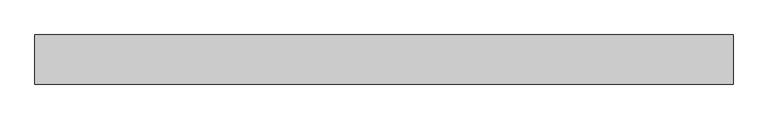
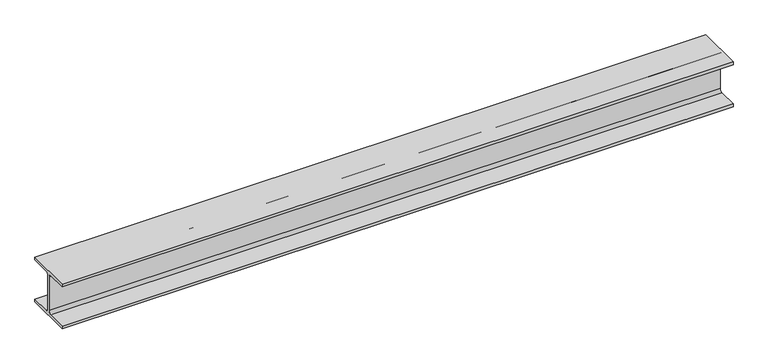
"""IFC4 building model written with IfcOpenShell, lengths in millimetres: beam geometry, 0912_Steel Framing_H-KSD3502 : H_SB_ASB_H-200x200x8x12."""

from ifc_helpers import new_model, si_unit, point, frame, frame_2d, origin, place, context, project, spatial, polyline, circle_curve, trimmed, segment, composite_curve, outline, extrude, source, transform, mapped, element, save


def beam_16896ac0(model_context):
    return source(origin(), model_context, "Body", "SweptSolid", [
        extrude(outline(composite_curve([segment(polyline([(100.0, -88.0), (100.0, -100.0), (-100.0, -100.0), (-100.0, -88.0), (-17.0, -88.0)]), True, "CONTINUOUS"), segment(trimmed(circle_curve(frame_2d((-17.0, -75.0)), 13.0), [point((-17.0, -88.0))], [point((-4.0, -75.0))], True, "CARTESIAN"), True, "CONTINUOUS"), segment(polyline([(-4.0, -75.0), (-4.0, 75.0)]), True, "CONTINUOUS"), segment(trimmed(circle_curve(frame_2d((-17.0, 75.0)), 13.0), [point((-4.0, 75.0))], [point((-17.0, 88.0))], True, "CARTESIAN"), True, "CONTINUOUS"), segment(polyline([(-17.0, 88.0), (-100.0, 88.0), (-100.0, 100.0), (100.0, 100.0), (100.0, 88.0), (17.0, 88.0)]), True, "CONTINUOUS"), segment(trimmed(circle_curve(frame_2d((17.0, 75.0)), 13.0), [point((17.0, 88.0))], [point((4.0, 75.0))], True, "CARTESIAN"), True, "CONTINUOUS"), segment(polyline([(4.0, 75.0), (4.0, -75.0)]), True, "CONTINUOUS"), segment(trimmed(circle_curve(frame_2d((17.0, -75.0)), 13.0), [point((4.0, -75.0))], [point((17.0, -88.0))], True, "CARTESIAN"), True, "CONTINUOUS"), segment(polyline([(17.0, -88.0), (100.0, -88.0)]), True, "CONTINUOUS")], self_intersect=False)), frame((-1433.1840333, 0.0, 0.0), z_axis=(1.0, 0.0, 0.0), x_axis=(0.0, 1.0, 0.0)), (0.0, 0.0, 1.0), 2842.115652),
    ])


if __name__ == "__main__":
    model = new_model("IFC4")
    model_context = context("Model", 3, world=origin())
    ifc_project = project(units=[si_unit("LENGTHUNIT", "METRE", prefix="MILLI")], contexts=[model_context])
    site = spatial("IfcSite", under=ifc_project)
    building = spatial("IfcBuilding", under=site)
    placement = place(None, origin())
    beam_shape = beam_16896ac0(model_context)
    element("IfcBeam", 1, ObjectType="0912_Steel Framing_H-KSD3502 : H_SB_ASB_H-200x200x8x12", at=placement, inside=building, context=model_context, shape_type="MappedRepresentation", body=[
        mapped(beam_shape, transform((0.0, 0.0, 0.0), x_axis=(1.0, 0.0, 0.0), y_axis=(0.0, 1.0, 0.0), z_axis=(0.0, 0.0, 1.0))),
    ])
    save(model, "model.ifc")

# Revit data of these elements
# Type "0912_Steel Framing_H-KSD3502 : H_SB_ASB_H-200x200x8x12"
#   H_WM Code_1 = "S01AA002-00001 | Main Steel Structure Fabrication Work | Shelter/Building | Medium Steel - Standard (90KG/M>Weight≥30KG/M) | Material: (   )"
#   H_WM Code_2 = "S03AA028-00001 | Main Steel Structure Erection Work | Shelter/Building | Medium Steel (90KG/M>Weight≥30KG/M) | Material: (   )"
#   H_WM Code_3 = "S01AA010-00001 | Main Steel Structure Fabrication Work | Shelter/Building | Steel Painting/Coating | for Non-Fireproofed Steel Surface, Surface Preparation, Primer, Second & Final Coat | Material: (   )"
#   H_Q'ty Cal Type Tag = "SB-Q2"
#   Width = 20.0 cm
#   Web Thickness = 0.8 cm
#   Web Fillet = 1.3 cm
#   Warping Constant = 141000.0 cm⁶
#   W = 0
#   Torsional Moment of Inertia = 26.2485 cm⁴
#   Section Area = 63.53 cm²
#   Plastic Modulus weak axis = 244.0 cm³
#   Plastic Modulus strong axis = 525.0 cm³
#   Perimeter = 1.16 m²/m
#   Nominal Weight = 49.90 kgf/m
#   Moment of Inertia weak axis = 1600.00 cm⁴
#   Moment of Inertia strong axis = 4720.00 cm⁴
#   Height = 20.0 cm
#   Flange Thickness = 1.2 cm
#   Elastic Modulus weak axis = 160.0 cm³
#   Elastic Modulus strong axis = 472.0 cm³
#   Centroid Vertical = 10.0 cm
#   Centroid Horizontal = 10.0 cm
#   Ix = 47200000
#   Length [instance default] = 1.5240 m
#   Zx = 525000
#   b = 0.2000 m
#   h = 0.2000 m
#   r = 0.0130 m
#   s = 0.0080 m
#   t = 0.0120 m
#   A = 0.006353 m²
#   Structural Material [instance default] = Steel, 45-345
#   Assembly Code = ""
# Element 1 (IfcBeam, "0912_Steel Framing_H-KSD3502 : H_SB_ASB_H-200x200x8x12")
#   Structural Material = none
# Materials
#   "Steel, 45-345": class "Metal", colour RGB 189 187 185, transparency 0, Description = "Steel 345 MPa", Cost = 0
